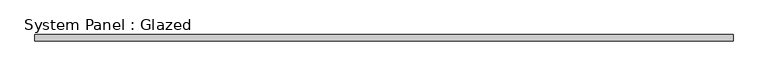
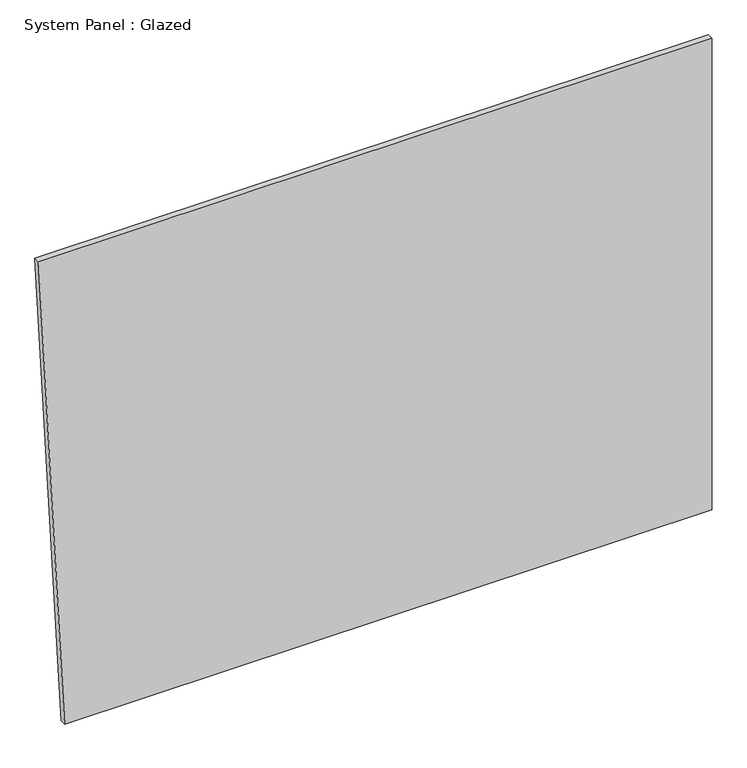
"""IFC4 building model written with IfcOpenShell, lengths in millimetres: plate geometry, System Panel : Glazed."""

from ifc_helpers import new_model, si_unit, frame, origin, place, context, project, spatial, polyline, outline, extrude, source, transform, mapped, element, save


def system_panel_glazed_fd15247c(model_context):
    return source(origin(), model_context, "Body", "SweptSolid", [
        extrude(outline(polyline([(0.0, -1299.9393804), (0.0, 1409.0796635), (2085.3785982, 1409.0796635), (2085.3785982, -1409.0796635), (0.0, -1299.9393804)])), frame((0.0, -44.45, 0.0), z_axis=(0.0, 1.0, 0.0), x_axis=(0.0, 0.0, 1.0)), (0.0, 0.0, 1.0), 25.4),
    ])


if __name__ == "__main__":
    model = new_model("IFC4")
    model_context = context("Model", 3, world=origin())
    ifc_project = project(units=[si_unit("LENGTHUNIT", "METRE", prefix="MILLI")], contexts=[model_context])
    site = spatial("IfcSite", under=ifc_project)
    building = spatial("IfcBuilding", under=site)
    placement = place(None, origin())
    system_panel_glazed_shape = system_panel_glazed_fd15247c(model_context)
    element("IfcPlate", 1, ObjectType="System Panel : Glazed", at=placement, inside=building, context=model_context, shape_type="MappedRepresentation", body=[
        mapped(system_panel_glazed_shape, transform((0.0, 0.0, 0.0), x_axis=(1.0, 0.0, 0.0), y_axis=(0.0, 1.0, 0.0), z_axis=(0.0, 0.0, 1.0))),
    ])
    save(model, "model.ifc")

# Revit data of these elements
# Type "System Panel : Glazed"
#   Construction Type Id = "GSP4R"
#   Analytic Construction = "1/8 in Pilkington single glazing"
#   Visual Light Transmittance = 0.9
#   Solar Heat Gain Coefficient = 0.86
#   Heat Transfer Coefficient (U) = 1.18115 BTU/(h·ft²·°F)
#   Define Thermal Properties by = 1
# Element 1 (IfcPlate, "System Panel : Glazed")
#   Materials on its faces: "Glass"
# Materials
#   "Glass": class "Glass", colour RGB 0 128 192, transparency 0.75, Description = "Soda Lime Glass", Cost = 0
